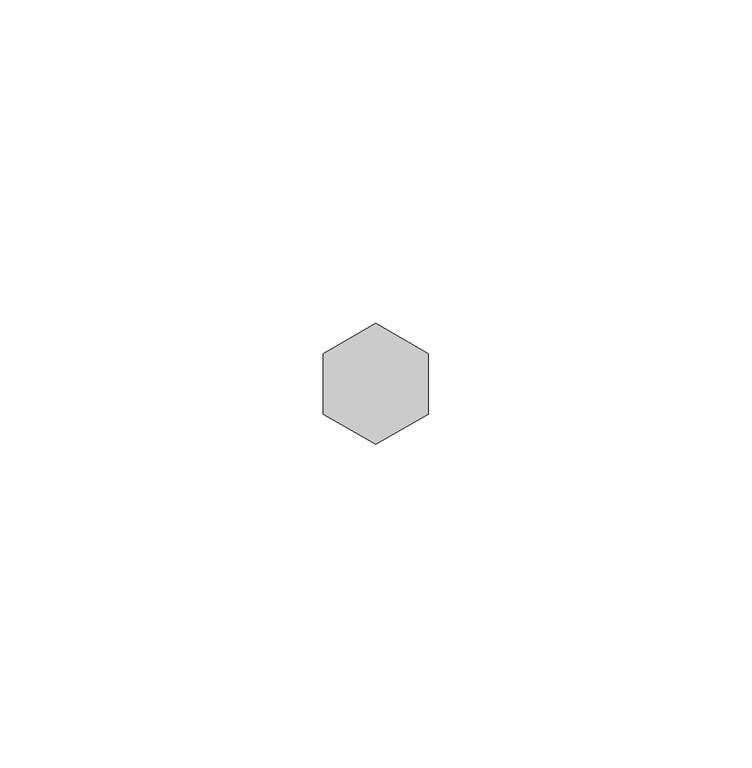
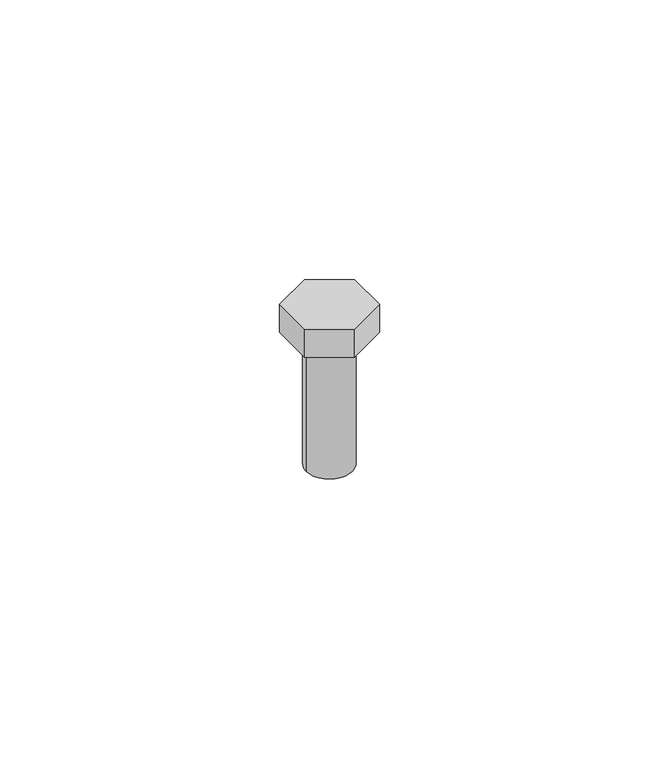
"""IFC4 building model written with IfcOpenShell, lengths in millimetres: proxy geometry, TN_Болт с шестигранной головкой (сборка) : Болт с шестигранной головкой (сборка тип 1)."""

import ifcopenshell
import ifcopenshell.guid

model = None  # the IFC model being written
_history = None  # IfcOwnerHistory: only IFC2X3 demands one
_inside = {}  # id of a spatial element -> (the spatial element, [elements in it])
_under = {}  # id of a project, library or spatial element -> (it, [spatial elements below it])
_declared = {}  # id of a project -> (the project, [libraries it declares])
_typed = {}  # id of a type object -> (the type object, [elements of that type])
_made_of = {}  # id of a material, layer set ... -> (it, [elements and type objects made of it])


def new_model(schema):
    """Start an empty IFC model of exactly this schema.

    Asked for "IFC4X3", IfcOpenShell would pick the latest addendum, in which some entities
    have other attributes; the version numbers below select the first issue.
    IFC2X3 requires an IfcOwnerHistory on every rooted entity: one is made here for all.
    """
    global model, _history
    if schema == "IFC4X3":
        model = ifcopenshell.file(schema_version=(4, 3, 0, 0))
    else:
        model = ifcopenshell.file(schema=schema)
    _inside.clear()
    _under.clear()
    _declared.clear()
    _typed.clear()
    _made_of.clear()
    _history = None
    if model.schema == "IFC2X3":
        org = make("IfcOrganization", Name="unknown")
        user = make(
            "IfcPersonAndOrganization",
            ThePerson=make("IfcPerson", FamilyName="unknown"),
            TheOrganization=org,
        )
        app = make(
            "IfcApplication",
            ApplicationDeveloper=org,
            Version="unknown",
            ApplicationFullName="unknown",
            ApplicationIdentifier="unknown",
        )
        _history = make(
            "IfcOwnerHistory",
            OwningUser=user,
            OwningApplication=app,
            ChangeAction="ADDED",
            CreationDate=0,
        )
    return model


def make(cls, **values):
    """One entity of the class cls with the attributes given. An attribute that is None is left unset."""
    return model.create_entity(
        cls, **{name: value for name, value in values.items() if value is not None}
    )


def rooted(cls, **values):
    """An entity with a GlobalId (a new one), such as an element, a storey or a relation."""
    return make(cls, GlobalId=ifcopenshell.guid.new(), OwnerHistory=_history, **values)


def si_unit(unit_type, name, prefix=None):
    """IfcSIUnit, for example si_unit("LENGTHUNIT", "METRE", prefix="MILLI")."""
    return make("IfcSIUnit", UnitType=unit_type, Prefix=prefix, Name=name)


def assignment(units):
    """IfcUnitAssignment: the units of a project."""
    return None if units is None else make("IfcUnitAssignment", Units=units)


def point(xyz):
    """IfcCartesianPoint."""
    return None if xyz is None else make("IfcCartesianPoint", Coordinates=xyz)


def direction(xyz):
    """IfcDirection."""
    return None if xyz is None else make("IfcDirection", DirectionRatios=xyz)


def frame(location, z_axis=None, x_axis=None):
    """IfcAxis2Placement3D, a coordinate frame: its origin and axes. An axis left out is left unset."""
    return make(
        "IfcAxis2Placement3D",
        Location=point(location),
        Axis=direction(z_axis),
        RefDirection=direction(x_axis),
    )


def frame_2d(location, x_axis=None):
    """IfcAxis2Placement2D, a coordinate frame in the plane: its origin and x axis."""
    return make(
        "IfcAxis2Placement2D", Location=point(location), RefDirection=direction(x_axis)
    )


def origin():
    """The frame at (0, 0, 0) with its axes left unset."""
    return frame((0.0, 0.0, 0.0))


def origin_with_axes():
    """The frame at (0, 0, 0) with the z axis (0, 0, 1) and the x axis (1, 0, 0) written out."""
    return frame((0.0, 0.0, 0.0), z_axis=(0.0, 0.0, 1.0), x_axis=(1.0, 0.0, 0.0))


def origin_2d():
    """The frame at (0, 0) in the plane with its x axis left unset."""
    return frame_2d((0.0, 0.0))


def place(relative_to, where):
    """IfcLocalPlacement: puts the frame where relative to a parent placement (None: the world)."""
    return make(
        "IfcLocalPlacement", PlacementRelTo=relative_to, RelativePlacement=where
    )


def context(
    kind, dimensions, precision=None, world=None, true_north=None, identifier=None
):
    """IfcGeometricRepresentationContext, for example the 3D "Model" context."""
    return make(
        "IfcGeometricRepresentationContext",
        ContextIdentifier=identifier,
        ContextType=kind,
        CoordinateSpaceDimension=dimensions,
        Precision=precision,
        WorldCoordinateSystem=world,
        TrueNorth=true_north,
    )


def project(units=None, contexts=None):
    """IfcProject with its units and contexts."""
    return rooted(
        "IfcProject",
        Name="project",
        RepresentationContexts=contexts,
        UnitsInContext=assignment(units),
    )


def spatial(cls, under=None, at=None, **own):
    """A site, building, storey or space (cls), placed at a placement, below another one or the project."""
    s = rooted(cls, ObjectPlacement=at, **own)
    if under is not None:
        _under.setdefault(under.id(), (under, []))[1].append(s)
    return s


def polyline(points):
    """IfcPolyline through the points."""
    return make("IfcPolyline", Points=[point(p) for p in points])


def circle_curve(where, radius):
    """IfcCircle in the frame where."""
    return make("IfcCircle", Position=where, Radius=radius)


def trimmed(basis, trim1, trim2, sense, master):
    """IfcTrimmedCurve: the piece of a basis curve between two trims."""
    return make(
        "IfcTrimmedCurve",
        BasisCurve=basis,
        Trim1=trim1,
        Trim2=trim2,
        SenseAgreement=sense,
        MasterRepresentation=master,
    )


def segment(curve, same_sense, transition):
    """IfcCompositeCurveSegment."""
    return make(
        "IfcCompositeCurveSegment",
        Transition=transition,
        SameSense=same_sense,
        ParentCurve=curve,
    )


def composite_curve(segments, self_intersect=None):
    """IfcCompositeCurve: segments joined end to end."""
    return make("IfcCompositeCurve", Segments=segments, SelfIntersect=self_intersect)


def outline(outer, holes=None, kind="AREA"):
    """IfcArbitraryClosedProfileDef: a profile drawn as a closed curve; with holes, ...WithVoids."""
    if holes is None:
        return make("IfcArbitraryClosedProfileDef", ProfileType=kind, OuterCurve=outer)
    return make(
        "IfcArbitraryProfileDefWithVoids",
        ProfileType=kind,
        OuterCurve=outer,
        InnerCurves=holes,
    )


def extrude(swept, where, along, depth):
    """IfcExtrudedAreaSolid: the profile swept, set in the frame where, extruded along a direction by depth."""
    return make(
        "IfcExtrudedAreaSolid",
        SweptArea=swept,
        Position=where,
        ExtrudedDirection=direction(along),
        Depth=depth,
    )


def shape(context_of_items, identifier, shape_type, items):
    """IfcShapeRepresentation: the items that make up one representation, for example the "Body"."""
    return make(
        "IfcShapeRepresentation",
        ContextOfItems=context_of_items,
        RepresentationIdentifier=identifier,
        RepresentationType=shape_type,
        Items=items,
    )


def source(mapping_origin, context_of_items, identifier, shape_type, items):
    """IfcRepresentationMap: a shape defined once, which mapped items show again and again."""
    return make(
        "IfcRepresentationMap",
        MappingOrigin=mapping_origin,
        MappedRepresentation=shape(context_of_items, identifier, shape_type, items),
    )


def transform(
    local_origin,
    x_axis=None,
    y_axis=None,
    z_axis=None,
    scale=None,
    scale2=None,
    scale3=None,
    uniform=True,
):
    """IfcCartesianTransformationOperator3D, or its non-uniform kind. x_axis, y_axis, z_axis: its Axis1, 2, 3."""
    if uniform:
        return make(
            "IfcCartesianTransformationOperator3D",
            Axis1=direction(x_axis),
            Axis2=direction(y_axis),
            LocalOrigin=point(local_origin),
            Scale=scale,
            Axis3=direction(z_axis),
        )
    return make(
        "IfcCartesianTransformationOperator3DnonUniform",
        Axis1=direction(x_axis),
        Axis2=direction(y_axis),
        LocalOrigin=point(local_origin),
        Scale=scale,
        Axis3=direction(z_axis),
        Scale2=scale2,
        Scale3=scale3,
    )


def mapped(mapping_source, mapping_target):
    """IfcMappedItem: shows the shape of a source again, moved by a transform."""
    return make(
        "IfcMappedItem", MappingSource=mapping_source, MappingTarget=mapping_target
    )


def made_of(thing, what):
    """Note that an element or type object is made of a material, layer set ...; save() writes the relation."""
    if what is not None:
        _made_of.setdefault(what.id(), (what, []))[1].append(thing)
    return thing


def element(
    cls,
    number,
    at=None,
    inside=None,
    cuts=None,
    type_object=None,
    material=None,
    context=None,
    identifier="Body",
    shape_type=None,
    held_by="IfcProductDefinitionShape",
    body=None,
    shapes=None,
    **own,
):
    """One element of the class cls, such as IfcWall. Its Tag is "e" and its number.

    at: its placement. inside: the storey or other place that contains it. cuts: it is an
    opening in that element (IfcRelVoidsElement). A single representation is given by context,
    identifier, shape_type and body (its items); several are given by shapes. held_by: the class
    of the entity that holds the representations. save() writes the other relations.
    """
    e = rooted(cls, Tag="e%d" % number, ObjectPlacement=at, **own)
    if body is not None:
        shapes = [shape(context, identifier, shape_type, body)]
    if shapes is not None:
        e.Representation = make(held_by, Representations=shapes)
    if inside is not None:
        _inside.setdefault(inside.id(), (inside, []))[1].append(e)
    if cuts is not None:
        rooted(
            "IfcRelVoidsElement", RelatingBuildingElement=cuts, RelatedOpeningElement=e
        )
    if type_object is not None:
        _typed.setdefault(type_object.id(), (type_object, []))[1].append(e)
    return made_of(e, material)


def aggregate(whole, parts):
    """IfcRelAggregates: a whole, such as a stair, and the parts it consists of."""
    return rooted("IfcRelAggregates", RelatingObject=whole, RelatedObjects=parts)


def save(model, path):
    """Write the relations noted so far, then the file.

    IfcRelAggregates (storeys below a building ...), IfcRelContainedInSpatialStructure (elements
    in a storey), IfcRelDefinesByType, IfcRelAssociatesMaterial and IfcRelDeclares: one each for
    every whole, place, type object, material and project.
    """
    for whole, parts in _under.values():
        aggregate(whole, parts)
    for where, things in _inside.values():
        rooted(
            "IfcRelContainedInSpatialStructure",
            RelatedElements=things,
            RelatingStructure=where,
        )
    for kind, things in _typed.values():
        rooted("IfcRelDefinesByType", RelatedObjects=things, RelatingType=kind)
    for what, things in _made_of.values():
        rooted("IfcRelAssociatesMaterial", RelatedObjects=things, RelatingMaterial=what)
    for by, libraries in _declared.values():
        rooted("IfcRelDeclares", RelatingContext=by, RelatedDefinitions=libraries)
    model.write(path)


def generic_models_6658c622(model_context):
    return source(origin(), model_context, "Body", "SweptSolid", [
        extrude(outline(polyline([(8.0973375, 4.675), (8.0973375, -4.675), (0.0, -9.35), (-8.0973375, -4.675), (-8.0973375, 4.675), (0.0, 9.35), (8.0973375, 4.675)])), origin_with_axes(), (0.0, 0.0, 1.0), 6.4),
        extrude(outline(composite_curve([segment(trimmed(circle_curve(origin_2d(), 5.0), [point((-5.0, 0.0))], [point((5.0, 0.0))], False, "CARTESIAN"), True, "CONTINUOUS"), segment(trimmed(circle_curve(origin_2d(), 5.0), [point((5.0, 0.0))], [point((-5.0, 0.0))], False, "CARTESIAN"), True, "CONTINUOUS")], self_intersect=False)), frame((0.0, 0.0, -30.0), z_axis=(0.0, 0.0, 1.0), x_axis=(1.0, 0.0, 0.0)), (0.0, 0.0, 1.0), 30.0),
    ])


if __name__ == "__main__":
    model = new_model("IFC4")
    model_context = context("Model", 3, world=origin())
    ifc_project = project(units=[si_unit("LENGTHUNIT", "METRE", prefix="MILLI")], contexts=[model_context])
    site = spatial("IfcSite", under=ifc_project)
    building = spatial("IfcBuilding", under=site)
    placement = place(None, origin())
    generic_models_shape = generic_models_6658c622(model_context)
    element("IfcBuildingElementProxy", 1, Name="TN_Болт с шестигранной головкой (сборка) : Болт с шестигранной головкой (сборка тип 1)", ObjectType="TN_Болт с шестигранной головкой (сборка) : Болт с шестигранной головкой (сборка тип 1)", at=placement, inside=building, context=model_context, shape_type="MappedRepresentation", body=[
        mapped(generic_models_shape, transform((0.0, 0.0, 0.0), x_axis=(1.0, 0.0, 0.0), y_axis=(0.0, 1.0, 0.0), z_axis=(0.0, 0.0, 1.0))),
    ])
    save(model, "model.ifc")

# Revit data of these elements
# Type "TN_Болт с шестигранной головкой (сборка) : Болт с шестигранной головкой (сборка тип 1)"
#   Description = "Обеспечивает прочное соединение нескольких деталей, соединение является разъемным. Качество болтового соединения обеспечивается качеством стали, классом прочности и формой болта.\r\nМатериал:\r\nСталь класс прочности 8,8 ГОСТ-7798 (DIN 933).\r\nГальваническое покрытие цинком."
#   Manufacturer = "ТехноНИКОЛЬ"
#   Model = "Комплектующие к опорам"
#   URL = "https://nav.tn.ru/knowledge-base/polimernye-membrany/opory-pod-oborudovanie-na-ploskoy-krovle/?sphrase_id=266812"
#   ADSK_Обозначение = "ТехноНИКОЛЬ"
#   ADSK_Наименование краткое = "M10x30"
#   ADSK_Наименование = "Болт с шестигранной головкой M10x30"
#   ADSK_Масса_Текст = ""
#   ADSK_Марка = "M10x30"
#   ADSK_Код изделия = "660826"
#   ADSK_Завод-изготовитель = "ТехноНИКОЛЬ"
#   ADSK_Единица измерения = "шт."
#   ADSK_Группирование = "Комплектующие к опорам"
#   ADSK_URL страницы изделия = "https://nav.tn.ru/knowledge-base/polimernye-membrany/opory-pod-oborudovanie-na-ploskoy-krovle/?sphrase_id=266812"
#   ADSK_URL документации изделия = ""
#   ADSK_Количество = 1
#   Гайка шестигранная DIN 934 M10 - 8 = no
#   Гайка быстрого монтажа потайная 41 8F M10 = yes
#   ADSK_Материал = TN_СтальГальванизированная_Серый
#   Default Elevation = 0
# Element 1 (IfcBuildingElementProxy, "TN_Болт с шестигранной головкой (сборка) : Болт с шестигранной головкой (сборка тип 1)")
#   Materials on its faces: "TN_СтальГальванизированная_Серый"
# Materials
#   "TN_СтальГальванизированная_Серый": class "Типовые", colour RGB 206 210 213, transparency 0, Cost = 0
